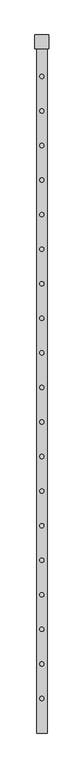
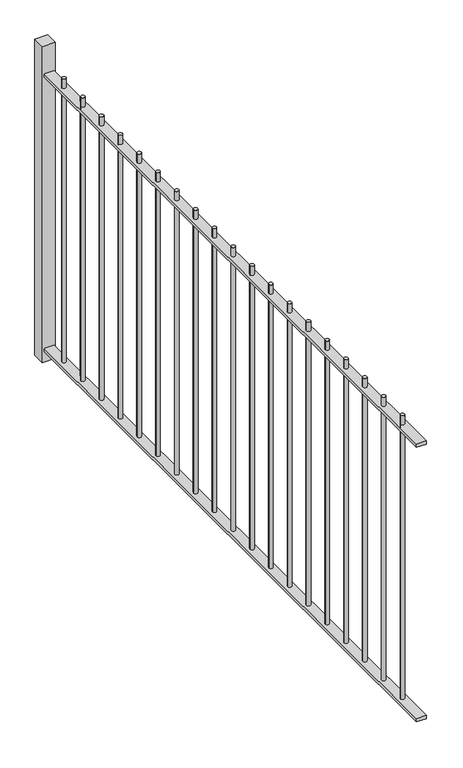
"""IFC4 building model written with IfcOpenShell, lengths in millimetres: railing geometry."""

from ifc_helpers import new_model, si_unit, point, frame, frame_2d, origin, place, context, project, spatial, polyline, circle_curve, trimmed, segment, composite_curve, outline, extrude, source, transform, mapped, element, save


def railing_1606a664(model_context):
    return source(origin(), model_context, "Body", "SweptSolid", [
        extrude(outline(polyline([(-6549.419961, 3348.8880881), (-6489.419961, 3348.8880881), (-6489.419961, -651.1119119), (-6549.419961, -651.1119119), (-6549.419961, 3348.8880881)])), frame((0.0, 0.0, -30.0), z_axis=(0.0, 0.0, 1.0), x_axis=(1.0, 0.0, 0.0)), (0.0, 0.0, 1.0), 20.0),
        extrude(outline(polyline([(-6549.419961, 3348.8880881), (-6489.419961, 3348.8880881), (-6489.419961, -651.1119119), (-6549.419961, -651.1119119), (-6549.419961, 3348.8880881)])), frame((0.0, 0.0, 1750.0), z_axis=(0.0, 0.0, 1.0), x_axis=(1.0, 0.0, 0.0)), (0.0, 0.0, 1.0), 20.0),
        extrude(outline(composite_curve([segment(trimmed(circle_curve(frame_2d((-6519.419961, -451.1119119)), 12.5), [point((-6531.919961, -451.1119119))], [point((-6506.919961, -451.1119119))], False, "CARTESIAN"), True, "CONTINUOUS"), segment(trimmed(circle_curve(frame_2d((-6519.419961, -451.1119119)), 12.5), [point((-6506.919961, -451.1119119))], [point((-6531.919961, -451.1119119))], False, "CARTESIAN"), True, "CONTINUOUS")], self_intersect=False)), frame((0.0, 0.0, -10.0), z_axis=(0.0, 0.0, 1.0), x_axis=(1.0, 0.0, 0.0)), (0.0, 0.0, 1.0), 1840.0),
        extrude(outline(composite_curve([segment(trimmed(circle_curve(frame_2d((-6519.419961, -251.1119119)), 12.5), [point((-6531.919961, -251.1119119))], [point((-6506.919961, -251.1119119))], False, "CARTESIAN"), True, "CONTINUOUS"), segment(trimmed(circle_curve(frame_2d((-6519.419961, -251.1119119)), 12.5), [point((-6506.919961, -251.1119119))], [point((-6531.919961, -251.1119119))], False, "CARTESIAN"), True, "CONTINUOUS")], self_intersect=False)), frame((0.0, 0.0, -10.0), z_axis=(0.0, 0.0, 1.0), x_axis=(1.0, 0.0, 0.0)), (0.0, 0.0, 1.0), 1840.0),
        extrude(outline(composite_curve([segment(trimmed(circle_curve(frame_2d((-6519.419961, -51.1119119)), 12.5), [point((-6531.919961, -51.1119119))], [point((-6506.919961, -51.1119119))], False, "CARTESIAN"), True, "CONTINUOUS"), segment(trimmed(circle_curve(frame_2d((-6519.419961, -51.1119119)), 12.5), [point((-6506.919961, -51.1119119))], [point((-6531.919961, -51.1119119))], False, "CARTESIAN"), True, "CONTINUOUS")], self_intersect=False)), frame((0.0, 0.0, -10.0), z_axis=(0.0, 0.0, 1.0), x_axis=(1.0, 0.0, 0.0)), (0.0, 0.0, 1.0), 1840.0),
        extrude(outline(composite_curve([segment(trimmed(circle_curve(frame_2d((-6519.419961, 148.8880881)), 12.5), [point((-6531.919961, 148.8880881))], [point((-6506.919961, 148.8880881))], False, "CARTESIAN"), True, "CONTINUOUS"), segment(trimmed(circle_curve(frame_2d((-6519.419961, 148.8880881)), 12.5), [point((-6506.919961, 148.8880881))], [point((-6531.919961, 148.8880881))], False, "CARTESIAN"), True, "CONTINUOUS")], self_intersect=False)), frame((0.0, 0.0, -10.0), z_axis=(0.0, 0.0, 1.0), x_axis=(1.0, 0.0, 0.0)), (0.0, 0.0, 1.0), 1840.0),
        extrude(outline(composite_curve([segment(trimmed(circle_curve(frame_2d((-6519.419961, 348.8880881)), 12.5), [point((-6531.919961, 348.8880881))], [point((-6506.919961, 348.8880881))], False, "CARTESIAN"), True, "CONTINUOUS"), segment(trimmed(circle_curve(frame_2d((-6519.419961, 348.8880881)), 12.5), [point((-6506.919961, 348.8880881))], [point((-6531.919961, 348.8880881))], False, "CARTESIAN"), True, "CONTINUOUS")], self_intersect=False)), frame((0.0, 0.0, -10.0), z_axis=(0.0, 0.0, 1.0), x_axis=(1.0, 0.0, 0.0)), (0.0, 0.0, 1.0), 1840.0),
        extrude(outline(composite_curve([segment(trimmed(circle_curve(frame_2d((-6519.419961, 548.8880881)), 12.5), [point((-6531.919961, 548.8880881))], [point((-6506.919961, 548.8880881))], False, "CARTESIAN"), True, "CONTINUOUS"), segment(trimmed(circle_curve(frame_2d((-6519.419961, 548.8880881)), 12.5), [point((-6506.919961, 548.8880881))], [point((-6531.919961, 548.8880881))], False, "CARTESIAN"), True, "CONTINUOUS")], self_intersect=False)), frame((0.0, 0.0, -10.0), z_axis=(0.0, 0.0, 1.0), x_axis=(1.0, 0.0, 0.0)), (0.0, 0.0, 1.0), 1840.0),
        extrude(outline(composite_curve([segment(trimmed(circle_curve(frame_2d((-6519.419961, 748.8880881)), 12.5), [point((-6531.919961, 748.8880881))], [point((-6506.919961, 748.8880881))], False, "CARTESIAN"), True, "CONTINUOUS"), segment(trimmed(circle_curve(frame_2d((-6519.419961, 748.8880881)), 12.5), [point((-6506.919961, 748.8880881))], [point((-6531.919961, 748.8880881))], False, "CARTESIAN"), True, "CONTINUOUS")], self_intersect=False)), frame((0.0, 0.0, -10.0), z_axis=(0.0, 0.0, 1.0), x_axis=(1.0, 0.0, 0.0)), (0.0, 0.0, 1.0), 1840.0),
        extrude(outline(composite_curve([segment(trimmed(circle_curve(frame_2d((-6519.419961, 948.8880881)), 12.5), [point((-6531.919961, 948.8880881))], [point((-6506.919961, 948.8880881))], False, "CARTESIAN"), True, "CONTINUOUS"), segment(trimmed(circle_curve(frame_2d((-6519.419961, 948.8880881)), 12.5), [point((-6506.919961, 948.8880881))], [point((-6531.919961, 948.8880881))], False, "CARTESIAN"), True, "CONTINUOUS")], self_intersect=False)), frame((0.0, 0.0, -10.0), z_axis=(0.0, 0.0, 1.0), x_axis=(1.0, 0.0, 0.0)), (0.0, 0.0, 1.0), 1840.0),
        extrude(outline(composite_curve([segment(trimmed(circle_curve(frame_2d((-6519.419961, 1148.8880881)), 12.5), [point((-6531.919961, 1148.8880881))], [point((-6506.919961, 1148.8880881))], False, "CARTESIAN"), True, "CONTINUOUS"), segment(trimmed(circle_curve(frame_2d((-6519.419961, 1148.8880881)), 12.5), [point((-6506.919961, 1148.8880881))], [point((-6531.919961, 1148.8880881))], False, "CARTESIAN"), True, "CONTINUOUS")], self_intersect=False)), frame((0.0, 0.0, -10.0), z_axis=(0.0, 0.0, 1.0), x_axis=(1.0, 0.0, 0.0)), (0.0, 0.0, 1.0), 1840.0),
        extrude(outline(composite_curve([segment(trimmed(circle_curve(frame_2d((-6519.419961, 1348.8880881)), 12.5), [point((-6531.919961, 1348.8880881))], [point((-6506.919961, 1348.8880881))], False, "CARTESIAN"), True, "CONTINUOUS"), segment(trimmed(circle_curve(frame_2d((-6519.419961, 1348.8880881)), 12.5), [point((-6506.919961, 1348.8880881))], [point((-6531.919961, 1348.8880881))], False, "CARTESIAN"), True, "CONTINUOUS")], self_intersect=False)), frame((0.0, 0.0, -10.0), z_axis=(0.0, 0.0, 1.0), x_axis=(1.0, 0.0, 0.0)), (0.0, 0.0, 1.0), 1840.0),
        extrude(outline(composite_curve([segment(trimmed(circle_curve(frame_2d((-6519.419961, 1548.8880881)), 12.5), [point((-6531.919961, 1548.8880881))], [point((-6506.919961, 1548.8880881))], False, "CARTESIAN"), True, "CONTINUOUS"), segment(trimmed(circle_curve(frame_2d((-6519.419961, 1548.8880881)), 12.5), [point((-6506.919961, 1548.8880881))], [point((-6531.919961, 1548.8880881))], False, "CARTESIAN"), True, "CONTINUOUS")], self_intersect=False)), frame((0.0, 0.0, -10.0), z_axis=(0.0, 0.0, 1.0), x_axis=(1.0, 0.0, 0.0)), (0.0, 0.0, 1.0), 1840.0),
        extrude(outline(composite_curve([segment(trimmed(circle_curve(frame_2d((-6519.419961, 1748.8880881)), 12.5), [point((-6531.919961, 1748.8880881))], [point((-6506.919961, 1748.8880881))], False, "CARTESIAN"), True, "CONTINUOUS"), segment(trimmed(circle_curve(frame_2d((-6519.419961, 1748.8880881)), 12.5), [point((-6506.919961, 1748.8880881))], [point((-6531.919961, 1748.8880881))], False, "CARTESIAN"), True, "CONTINUOUS")], self_intersect=False)), frame((0.0, 0.0, -10.0), z_axis=(0.0, 0.0, 1.0), x_axis=(1.0, 0.0, 0.0)), (0.0, 0.0, 1.0), 1840.0),
        extrude(outline(composite_curve([segment(trimmed(circle_curve(frame_2d((-6519.419961, 1948.8880881)), 12.5), [point((-6531.919961, 1948.8880881))], [point((-6506.919961, 1948.8880881))], False, "CARTESIAN"), True, "CONTINUOUS"), segment(trimmed(circle_curve(frame_2d((-6519.419961, 1948.8880881)), 12.5), [point((-6506.919961, 1948.8880881))], [point((-6531.919961, 1948.8880881))], False, "CARTESIAN"), True, "CONTINUOUS")], self_intersect=False)), frame((0.0, 0.0, -10.0), z_axis=(0.0, 0.0, 1.0), x_axis=(1.0, 0.0, 0.0)), (0.0, 0.0, 1.0), 1840.0),
        extrude(outline(composite_curve([segment(trimmed(circle_curve(frame_2d((-6519.419961, 2148.8880881)), 12.5), [point((-6531.919961, 2148.8880881))], [point((-6506.919961, 2148.8880881))], False, "CARTESIAN"), True, "CONTINUOUS"), segment(trimmed(circle_curve(frame_2d((-6519.419961, 2148.8880881)), 12.5), [point((-6506.919961, 2148.8880881))], [point((-6531.919961, 2148.8880881))], False, "CARTESIAN"), True, "CONTINUOUS")], self_intersect=False)), frame((0.0, 0.0, -10.0), z_axis=(0.0, 0.0, 1.0), x_axis=(1.0, 0.0, 0.0)), (0.0, 0.0, 1.0), 1840.0),
        extrude(outline(composite_curve([segment(trimmed(circle_curve(frame_2d((-6519.419961, 2348.8880881)), 12.5), [point((-6531.919961, 2348.8880881))], [point((-6506.919961, 2348.8880881))], False, "CARTESIAN"), True, "CONTINUOUS"), segment(trimmed(circle_curve(frame_2d((-6519.419961, 2348.8880881)), 12.5), [point((-6506.919961, 2348.8880881))], [point((-6531.919961, 2348.8880881))], False, "CARTESIAN"), True, "CONTINUOUS")], self_intersect=False)), frame((0.0, 0.0, -10.0), z_axis=(0.0, 0.0, 1.0), x_axis=(1.0, 0.0, 0.0)), (0.0, 0.0, 1.0), 1840.0),
        extrude(outline(composite_curve([segment(trimmed(circle_curve(frame_2d((-6519.419961, 2548.8880881)), 12.5), [point((-6531.919961, 2548.8880881))], [point((-6506.919961, 2548.8880881))], False, "CARTESIAN"), True, "CONTINUOUS"), segment(trimmed(circle_curve(frame_2d((-6519.419961, 2548.8880881)), 12.5), [point((-6506.919961, 2548.8880881))], [point((-6531.919961, 2548.8880881))], False, "CARTESIAN"), True, "CONTINUOUS")], self_intersect=False)), frame((0.0, 0.0, -10.0), z_axis=(0.0, 0.0, 1.0), x_axis=(1.0, 0.0, 0.0)), (0.0, 0.0, 1.0), 1840.0),
        extrude(outline(composite_curve([segment(trimmed(circle_curve(frame_2d((-6519.419961, 2748.8880881)), 12.5), [point((-6531.919961, 2748.8880881))], [point((-6506.919961, 2748.8880881))], False, "CARTESIAN"), True, "CONTINUOUS"), segment(trimmed(circle_curve(frame_2d((-6519.419961, 2748.8880881)), 12.5), [point((-6506.919961, 2748.8880881))], [point((-6531.919961, 2748.8880881))], False, "CARTESIAN"), True, "CONTINUOUS")], self_intersect=False)), frame((0.0, 0.0, -10.0), z_axis=(0.0, 0.0, 1.0), x_axis=(1.0, 0.0, 0.0)), (0.0, 0.0, 1.0), 1840.0),
        extrude(outline(composite_curve([segment(trimmed(circle_curve(frame_2d((-6519.419961, 2948.8880881)), 12.5), [point((-6531.919961, 2948.8880881))], [point((-6506.919961, 2948.8880881))], False, "CARTESIAN"), True, "CONTINUOUS"), segment(trimmed(circle_curve(frame_2d((-6519.419961, 2948.8880881)), 12.5), [point((-6506.919961, 2948.8880881))], [point((-6531.919961, 2948.8880881))], False, "CARTESIAN"), True, "CONTINUOUS")], self_intersect=False)), frame((0.0, 0.0, -10.0), z_axis=(0.0, 0.0, 1.0), x_axis=(1.0, 0.0, 0.0)), (0.0, 0.0, 1.0), 1840.0),
        extrude(outline(composite_curve([segment(trimmed(circle_curve(frame_2d((-6519.419961, 3148.8880881)), 12.5), [point((-6531.919961, 3148.8880881))], [point((-6506.919961, 3148.8880881))], False, "CARTESIAN"), True, "CONTINUOUS"), segment(trimmed(circle_curve(frame_2d((-6519.419961, 3148.8880881)), 12.5), [point((-6506.919961, 3148.8880881))], [point((-6531.919961, 3148.8880881))], False, "CARTESIAN"), True, "CONTINUOUS")], self_intersect=False)), frame((0.0, 0.0, -10.0), z_axis=(0.0, 0.0, 1.0), x_axis=(1.0, 0.0, 0.0)), (0.0, 0.0, 1.0), 1840.0),
        extrude(outline(polyline([(-6479.419961, 3388.8880881), (-6479.419961, 3308.8880881), (-6559.419961, 3308.8880881), (-6559.419961, 3388.8880881), (-6479.419961, 3388.8880881)])), frame((0.0, 0.0, -100.0), z_axis=(0.0, 0.0, 1.0), x_axis=(1.0, 0.0, 0.0)), (0.0, 0.0, 1.0), 2050.0),
    ])


if __name__ == "__main__":
    model = new_model("IFC4")
    model_context = context("Model", 3, world=origin())
    ifc_project = project(units=[si_unit("LENGTHUNIT", "METRE", prefix="MILLI")], contexts=[model_context])
    site = spatial("IfcSite", under=ifc_project)
    building = spatial("IfcBuilding", under=site)
    placement = place(None, origin())
    railing_shape = railing_1606a664(model_context)
    element("IfcRailing", 1, at=placement, inside=building, context=model_context, shape_type="MappedRepresentation", body=[
        mapped(railing_shape, transform((0.0, 0.0, 0.0), x_axis=(1.0, 0.0, 0.0), y_axis=(0.0, 1.0, 0.0), z_axis=(0.0, 0.0, 1.0))),
    ])
    save(model, "model.ifc")

# Revit data of these elements
# Element 1 (IfcRailing)
#   Materials on its faces: "NLRS_h2_staal_generiek zwart_gen_rsf", "NLRS_h2_staal_gen_rsf"
# Materials
#   "NLRS_h2_staal_generiek zwart_gen_rsf": class "Metal", colour RGB 189 187 185, transparency 0, Manufacturer = "RevitGG", URL = "www.revitgg.nl", Description = "Staal, generiek materiaal", Cost = 0
#   "NLRS_h2_staal_gen_rsf": class "H - Metaal", colour RGB 189 187 185, transparency 0, Keynote = "h2", Model = "generiek", Manufacturer = "Revit Standards Foundation", URL = "www.revitstandards.org", Description = "staal", Cost = 0
